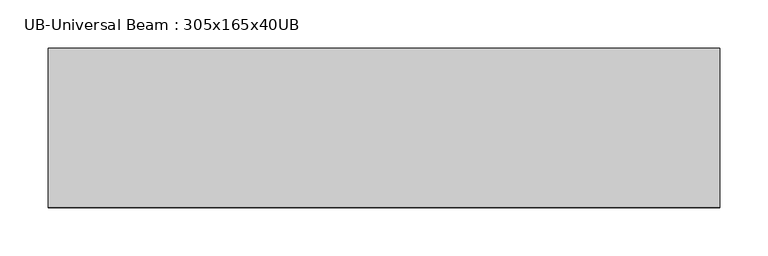
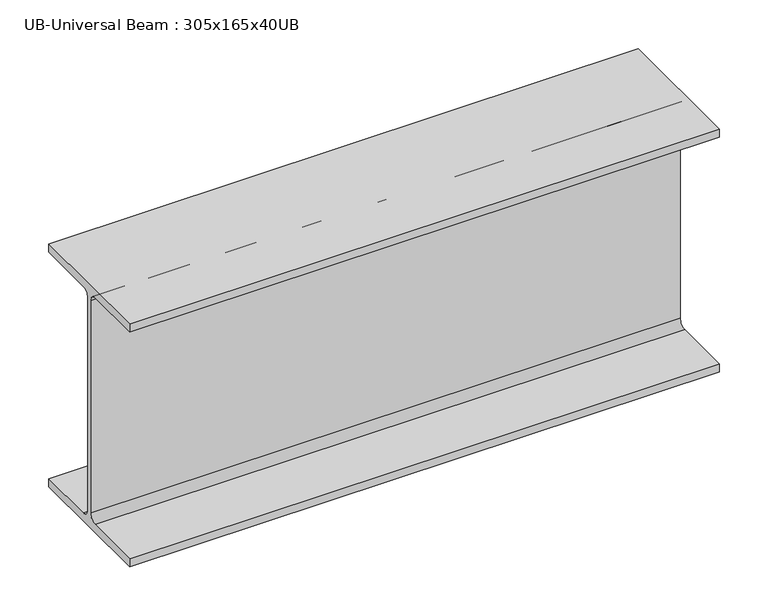
"""IFC4 building model written with IfcOpenShell, lengths in millimetres: beam geometry, UB-Universal Beam : 305x165x40UB."""

from ifc_helpers import new_model, si_unit, point, frame, frame_2d, origin, place, context, project, spatial, polyline, circle_curve, trimmed, segment, composite_curve, outline, extrude, source, transform, mapped, element, save


def ub_universal_beam_305x165x40ub_26fb8d3a(model_context):
    return source(origin(), model_context, "Body", "SweptSolid", [
        extrude(outline(composite_curve([segment(polyline([(82.5, -141.5), (82.5, -151.7), (-82.5, -151.7), (-82.5, -141.5), (-11.9, -141.5)]), True, "CONTINUOUS"), segment(trimmed(circle_curve(frame_2d((-11.9, -132.6)), 8.9), [point((-11.9, -141.5))], [point((-3.0, -132.6))], True, "CARTESIAN"), True, "CONTINUOUS"), segment(polyline([(-3.0, -132.6), (-3.0, 132.6)]), True, "CONTINUOUS"), segment(trimmed(circle_curve(frame_2d((-11.9, 132.6)), 8.9), [point((-3.0, 132.6))], [point((-11.9, 141.5))], True, "CARTESIAN"), True, "CONTINUOUS"), segment(polyline([(-11.9, 141.5), (-82.5, 141.5), (-82.5, 151.7), (82.5, 151.7), (82.5, 141.5), (11.9, 141.5)]), True, "CONTINUOUS"), segment(trimmed(circle_curve(frame_2d((11.9, 132.6)), 8.9), [point((11.9, 141.5))], [point((3.0, 132.6))], True, "CARTESIAN"), True, "CONTINUOUS"), segment(polyline([(3.0, 132.6), (3.0, -132.6)]), True, "CONTINUOUS"), segment(trimmed(circle_curve(frame_2d((11.9, -132.6)), 8.9), [point((3.0, -132.6))], [point((11.9, -141.5))], True, "CARTESIAN"), True, "CONTINUOUS"), segment(polyline([(11.9, -141.5), (82.5, -141.5)]), True, "CONTINUOUS")], self_intersect=False)), frame((-347.8807825, 0.0, 0.0), z_axis=(1.0, 0.0, 0.0), x_axis=(0.0, 1.0, 0.0)), (0.0, 0.0, 1.0), 695.761565),
    ])


if __name__ == "__main__":
    model = new_model("IFC4")
    model_context = context("Model", 3, world=origin())
    ifc_project = project(units=[si_unit("LENGTHUNIT", "METRE", prefix="MILLI")], contexts=[model_context])
    site = spatial("IfcSite", under=ifc_project)
    building = spatial("IfcBuilding", under=site)
    placement = place(None, origin())
    ub_universal_beam_305x165x40ub_shape = ub_universal_beam_305x165x40ub_26fb8d3a(model_context)
    element("IfcBeam", 1, ObjectType="UB-Universal Beam : 305x165x40UB", at=placement, inside=building, context=model_context, shape_type="MappedRepresentation", body=[
        mapped(ub_universal_beam_305x165x40ub_shape, transform((0.0, 0.0, 0.0), x_axis=(1.0, 0.0, 0.0), y_axis=(0.0, 1.0, 0.0), z_axis=(0.0, 0.0, 1.0))),
    ])
    save(model, "model.ifc")

# Revit data of these elements
# Type "UB-Universal Beam : 305x165x40UB"
#   Nominal h = "305"
#   W = 0
#   Start Extension Calculation [instance default] = 3000 mm
#   Start Extension [instance default] = -12.7 mm
#   End Extension Calculation [instance default] = 3000 mm
#   End Extension [instance default] = -12.7 mm
#   Ix = 8503
#   Length [instance default] = 1524 mm
#   M = 40.3
#   Zx = 560
#   b = 165 mm
#   h = 303.4 mm
#   r = 8.9 mm
#   s = 6 mm
#   t = 10.2 mm
#   A = 0.005 m²
#   Structural Material [instance default] = Metal - Steel - 345 MPa
#   Assembly Code = ""
# Element 1 (IfcBeam, "UB-Universal Beam : 305x165x40UB")
#   Materials on its faces: "Metal - Steel - 345 MPa"
# Materials
#   "Metal - Steel - 345 MPa": class "Metal", colour RGB 241 46 46, transparency 0
